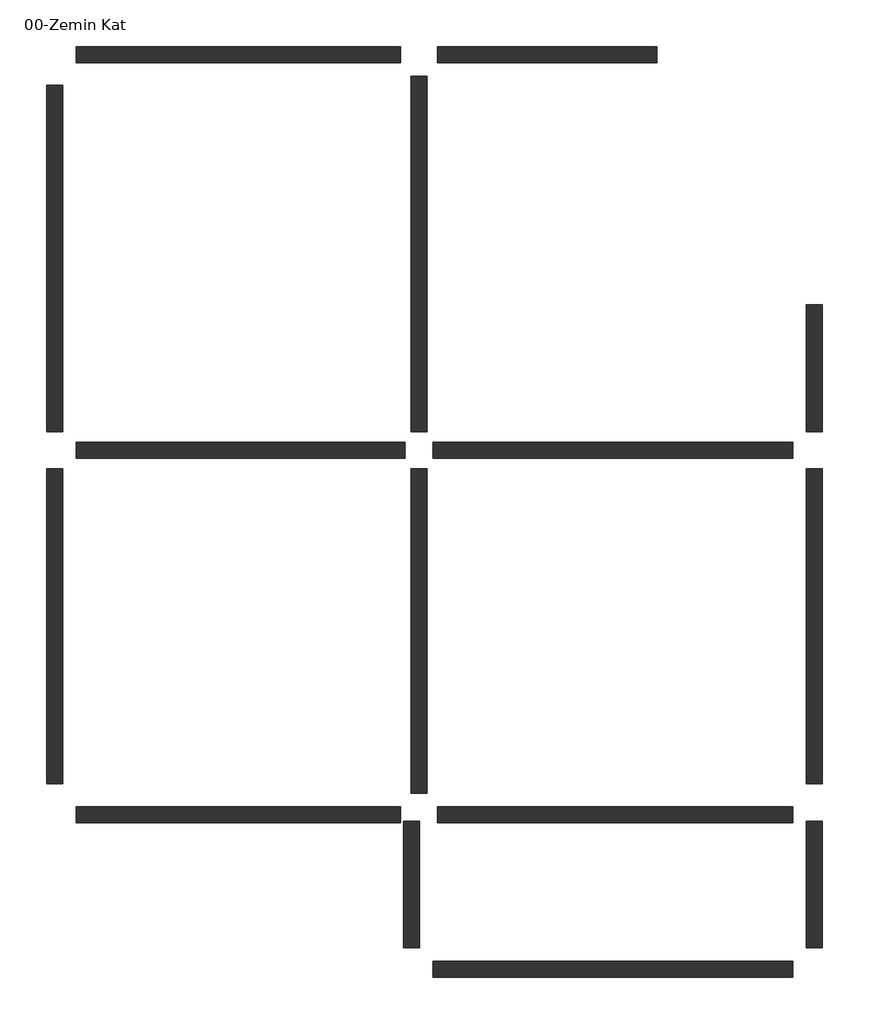
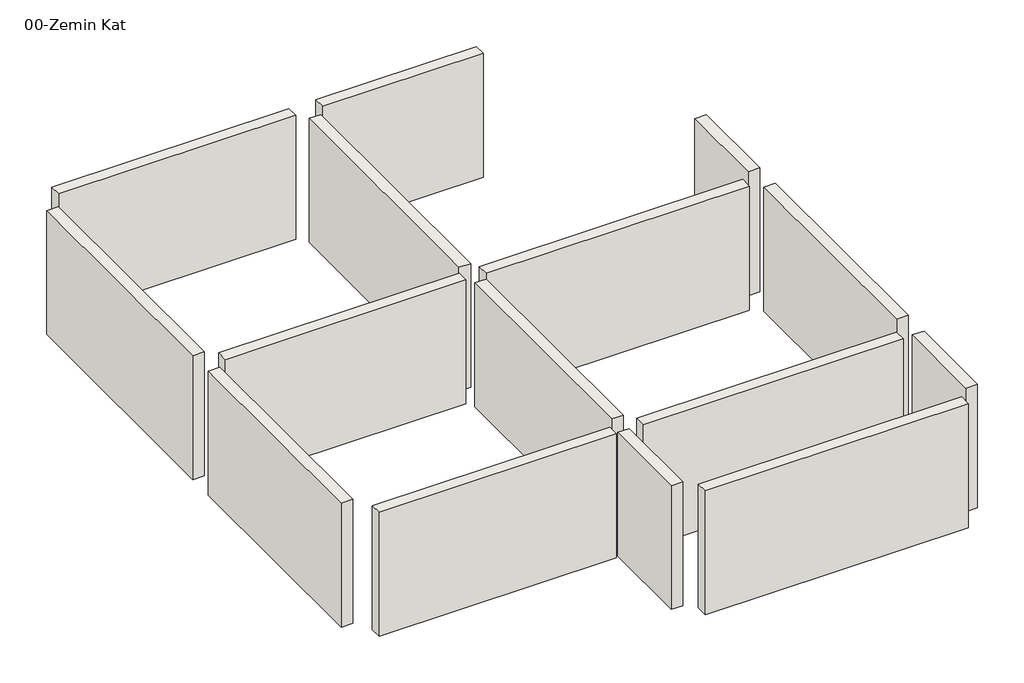
# One storey: 15 walls.
"""IFC4 building model written with IfcOpenShell, lengths in millimetres."""

import ifcopenshell
import ifcopenshell.guid

model = None  # the IFC model being written
_history = None  # IfcOwnerHistory: only IFC2X3 demands one
_inside = {}  # id of a spatial element -> (the spatial element, [elements in it])
_under = {}  # id of a project, library or spatial element -> (it, [spatial elements below it])
_declared = {}  # id of a project -> (the project, [libraries it declares])
_typed = {}  # id of a type object -> (the type object, [elements of that type])
_made_of = {}  # id of a material, layer set ... -> (it, [elements and type objects made of it])


def new_model(schema):
    """Start an empty IFC model of exactly this schema.

    Asked for "IFC4X3", IfcOpenShell would pick the latest addendum, in which some entities
    have other attributes; the version numbers below select the first issue.
    IFC2X3 requires an IfcOwnerHistory on every rooted entity: one is made here for all.
    """
    global model, _history
    if schema == "IFC4X3":
        model = ifcopenshell.file(schema_version=(4, 3, 0, 0))
    else:
        model = ifcopenshell.file(schema=schema)
    _inside.clear()
    _under.clear()
    _declared.clear()
    _typed.clear()
    _made_of.clear()
    _history = None
    if model.schema == "IFC2X3":
        org = make("IfcOrganization", Name="unknown")
        user = make(
            "IfcPersonAndOrganization",
            ThePerson=make("IfcPerson", FamilyName="unknown"),
            TheOrganization=org,
        )
        app = make(
            "IfcApplication",
            ApplicationDeveloper=org,
            Version="unknown",
            ApplicationFullName="unknown",
            ApplicationIdentifier="unknown",
        )
        _history = make(
            "IfcOwnerHistory",
            OwningUser=user,
            OwningApplication=app,
            ChangeAction="ADDED",
            CreationDate=0,
        )
    return model


def make(cls, **values):
    """One entity of the class cls with the attributes given. An attribute that is None is left unset."""
    return model.create_entity(
        cls, **{name: value for name, value in values.items() if value is not None}
    )


def rooted(cls, **values):
    """An entity with a GlobalId (a new one), such as an element, a storey or a relation."""
    return make(cls, GlobalId=ifcopenshell.guid.new(), OwnerHistory=_history, **values)


def si_unit(unit_type, name, prefix=None):
    """IfcSIUnit, for example si_unit("LENGTHUNIT", "METRE", prefix="MILLI")."""
    return make("IfcSIUnit", UnitType=unit_type, Prefix=prefix, Name=name)


def assignment(units):
    """IfcUnitAssignment: the units of a project."""
    return None if units is None else make("IfcUnitAssignment", Units=units)


def point(xyz):
    """IfcCartesianPoint."""
    return None if xyz is None else make("IfcCartesianPoint", Coordinates=xyz)


def direction(xyz):
    """IfcDirection."""
    return None if xyz is None else make("IfcDirection", DirectionRatios=xyz)


def frame(location, z_axis=None, x_axis=None):
    """IfcAxis2Placement3D, a coordinate frame: its origin and axes. An axis left out is left unset."""
    return make(
        "IfcAxis2Placement3D",
        Location=point(location),
        Axis=direction(z_axis),
        RefDirection=direction(x_axis),
    )


def origin():
    """The frame at (0, 0, 0) with its axes left unset."""
    return frame((0.0, 0.0, 0.0))


def place(relative_to, where):
    """IfcLocalPlacement: puts the frame where relative to a parent placement (None: the world)."""
    return make(
        "IfcLocalPlacement", PlacementRelTo=relative_to, RelativePlacement=where
    )


def context(
    kind, dimensions, precision=None, world=None, true_north=None, identifier=None
):
    """IfcGeometricRepresentationContext, for example the 3D "Model" context."""
    return make(
        "IfcGeometricRepresentationContext",
        ContextIdentifier=identifier,
        ContextType=kind,
        CoordinateSpaceDimension=dimensions,
        Precision=precision,
        WorldCoordinateSystem=world,
        TrueNorth=true_north,
    )


def project(units=None, contexts=None):
    """IfcProject with its units and contexts."""
    return rooted(
        "IfcProject",
        Name="project",
        RepresentationContexts=contexts,
        UnitsInContext=assignment(units),
    )


def spatial(cls, under=None, at=None, **own):
    """A site, building, storey or space (cls), placed at a placement, below another one or the project."""
    s = rooted(cls, ObjectPlacement=at, **own)
    if under is not None:
        _under.setdefault(under.id(), (under, []))[1].append(s)
    return s


def polyline(points):
    """IfcPolyline through the points."""
    return make("IfcPolyline", Points=[point(p) for p in points])


def outline(outer, holes=None, kind="AREA"):
    """IfcArbitraryClosedProfileDef: a profile drawn as a closed curve; with holes, ...WithVoids."""
    if holes is None:
        return make("IfcArbitraryClosedProfileDef", ProfileType=kind, OuterCurve=outer)
    return make(
        "IfcArbitraryProfileDefWithVoids",
        ProfileType=kind,
        OuterCurve=outer,
        InnerCurves=holes,
    )


def extrude(swept, where, along, depth):
    """IfcExtrudedAreaSolid: the profile swept, set in the frame where, extruded along a direction by depth."""
    return make(
        "IfcExtrudedAreaSolid",
        SweptArea=swept,
        Position=where,
        ExtrudedDirection=direction(along),
        Depth=depth,
    )


def shape(context_of_items, identifier, shape_type, items):
    """IfcShapeRepresentation: the items that make up one representation, for example the "Body"."""
    return make(
        "IfcShapeRepresentation",
        ContextOfItems=context_of_items,
        RepresentationIdentifier=identifier,
        RepresentationType=shape_type,
        Items=items,
    )


def made_of(thing, what):
    """Note that an element or type object is made of a material, layer set ...; save() writes the relation."""
    if what is not None:
        _made_of.setdefault(what.id(), (what, []))[1].append(thing)
    return thing


def element(
    cls,
    number,
    at=None,
    inside=None,
    cuts=None,
    type_object=None,
    material=None,
    context=None,
    identifier="Body",
    shape_type=None,
    held_by="IfcProductDefinitionShape",
    body=None,
    shapes=None,
    **own,
):
    """One element of the class cls, such as IfcWall. Its Tag is "e" and its number.

    at: its placement. inside: the storey or other place that contains it. cuts: it is an
    opening in that element (IfcRelVoidsElement). A single representation is given by context,
    identifier, shape_type and body (its items); several are given by shapes. held_by: the class
    of the entity that holds the representations. save() writes the other relations.
    """
    e = rooted(cls, Tag="e%d" % number, ObjectPlacement=at, **own)
    if body is not None:
        shapes = [shape(context, identifier, shape_type, body)]
    if shapes is not None:
        e.Representation = make(held_by, Representations=shapes)
    if inside is not None:
        _inside.setdefault(inside.id(), (inside, []))[1].append(e)
    if cuts is not None:
        rooted(
            "IfcRelVoidsElement", RelatingBuildingElement=cuts, RelatedOpeningElement=e
        )
    if type_object is not None:
        _typed.setdefault(type_object.id(), (type_object, []))[1].append(e)
    return made_of(e, material)


def aggregate(whole, parts):
    """IfcRelAggregates: a whole, such as a stair, and the parts it consists of."""
    return rooted("IfcRelAggregates", RelatingObject=whole, RelatedObjects=parts)


def save(model, path):
    """Write the relations noted so far, then the file.

    IfcRelAggregates (storeys below a building ...), IfcRelContainedInSpatialStructure (elements
    in a storey), IfcRelDefinesByType, IfcRelAssociatesMaterial and IfcRelDeclares: one each for
    every whole, place, type object, material and project.
    """
    for whole, parts in _under.values():
        aggregate(whole, parts)
    for where, things in _inside.values():
        rooted(
            "IfcRelContainedInSpatialStructure",
            RelatedElements=things,
            RelatingStructure=where,
        )
    for kind, things in _typed.values():
        rooted("IfcRelDefinesByType", RelatedObjects=things, RelatingType=kind)
    for what, things in _made_of.values():
        rooted("IfcRelAssociatesMaterial", RelatedObjects=things, RelatingMaterial=what)
    for by, libraries in _declared.values():
        rooted("IfcRelDeclares", RelatingContext=by, RelatedDefinitions=libraries)
    model.write(path)


model = new_model("IFC4")

# Units and contexts
model_context = context("Model", 3, world=origin())
ifc_project = project(units=[si_unit("LENGTHUNIT", "METRE", prefix="MILLI")], contexts=[model_context])

# Site, building, storey
site = spatial("IfcSite", under=ifc_project)
building = spatial("IfcBuilding", under=site)
storey = spatial("IfcBuildingStorey", under=building, Name="00-Zemin Kat", Elevation=93780.0)

# Walls
placement = place(None, origin())
element("IfcWall", 1, ObjectType="1.5BY-1.5SV-20BR-1.5-1.5BY", at=placement, inside=storey, context=model_context, shape_type="SweptSolid", body=[
    extrude(outline(polyline([(5700.0, 14770.0), (450.0, 14770.0), (450.0, 15030.0), (5700.0, 15030.0), (5700.0, 14770.0)])), frame((0.0, 0.0, 93780.0), z_axis=(0.0, 0.0, 1.0), x_axis=(1.0, 0.0, 0.0)), (0.0, 0.0, 1.0), 2900.0),
])
element("IfcWall", 2, ObjectType="1.5BY-1.5SV-20BR-1.5-1.5BY", at=placement, inside=storey, context=model_context, shape_type="SweptSolid", body=[
    extrude(outline(polyline([(9850.0, 14770.0), (6300.0, 14770.0), (6300.0, 15030.0), (9850.0, 15030.0), (9850.0, 14770.0)])), frame((0.0, 0.0, 93780.0), z_axis=(0.0, 0.0, 1.0), x_axis=(1.0, 0.0, 0.0)), (0.0, 0.0, 1.0), 2900.0),
])
element("IfcWall", 3, ObjectType="1.5BY-1.5SV-20BR-1.5-1.5BY", at=placement, inside=storey, context=model_context, shape_type="SweptSolid", body=[
    extrude(outline(polyline([(12270.0, 8800.0), (12270.0, 10850.0), (12530.0, 10850.0), (12530.0, 8800.0), (12270.0, 8800.0)])), frame((0.0, 0.0, 93780.0), z_axis=(0.0, 0.0, 1.0), x_axis=(1.0, 0.0, 0.0)), (0.0, 0.0, 1.0), 2900.0),
])
element("IfcWall", 4, ObjectType="1.5BY-1.5SV-20BR-1.5-1.5BY", at=placement, inside=storey, context=model_context, shape_type="SweptSolid", body=[
    extrude(outline(polyline([(12270.0, 3100.0), (12270.0, 8200.0), (12530.0, 8200.0), (12530.0, 3100.0), (12270.0, 3100.0)])), frame((0.0, 0.0, 93780.0), z_axis=(0.0, 0.0, 1.0), x_axis=(1.0, 0.0, 0.0)), (0.0, 0.0, 1.0), 2900.0),
])
element("IfcWall", 5, ObjectType="1.5BY-1.5SV-20BR-1.5-1.5BY", at=placement, inside=storey, context=model_context, shape_type="SweptSolid", body=[
    extrude(outline(polyline([(12270.0, 450.0), (12270.0, 2500.0), (12530.0, 2500.0), (12530.0, 450.0), (12270.0, 450.0)])), frame((0.0, 0.0, 93780.0), z_axis=(0.0, 0.0, 1.0), x_axis=(1.0, 0.0, 0.0)), (0.0, 0.0, 1.0), 2900.0),
])
element("IfcWall", 6, ObjectType="1.5BY-1.5SV-20BR-1.5-1.5BY", at=placement, inside=storey, context=model_context, shape_type="SweptSolid", body=[
    extrude(outline(polyline([(6225.0, 230.0), (12050.0, 230.0), (12050.0, -30.0), (6225.0, -30.0), (6225.0, 230.0)])), frame((0.0, 0.0, 93780.0), z_axis=(0.0, 0.0, 1.0), x_axis=(1.0, 0.0, 0.0)), (0.0, 0.0, 1.0), 2900.0),
])
element("IfcWall", 7, ObjectType="1.5BY-1.5SV-20BR-1.5-1.5BY", at=placement, inside=storey, context=model_context, shape_type="SweptSolid", body=[
    extrude(outline(polyline([(6005.0, 2500.0), (6005.0, 450.0), (5745.0, 450.0), (5745.0, 2500.0), (6005.0, 2500.0)])), frame((0.0, 0.0, 93780.0), z_axis=(0.0, 0.0, 1.0), x_axis=(1.0, 0.0, 0.0)), (0.0, 0.0, 1.0), 2900.0),
])
element("IfcWall", 8, ObjectType="1.5BY-1.5SV-20BR-1.5-1.5BY", at=placement, inside=storey, context=model_context, shape_type="SweptSolid", body=[
    extrude(outline(polyline([(450.0, 2730.0), (5700.0, 2730.0), (5700.0, 2470.0), (450.0, 2470.0), (450.0, 2730.0)])), frame((0.0, 0.0, 93780.0), z_axis=(0.0, 0.0, 1.0), x_axis=(1.0, 0.0, 0.0)), (0.0, 0.0, 1.0), 2900.0),
])
element("IfcWall", 9, ObjectType="1.5BY-1.5SV-20BR-1.5-1.5BY", at=placement, inside=storey, context=model_context, shape_type="SweptSolid", body=[
    extrude(outline(polyline([(230.0, 8200.0), (230.0, 3100.0), (-30.0, 3100.0), (-30.0, 8200.0), (230.0, 8200.0)])), frame((0.0, 0.0, 93780.0), z_axis=(0.0, 0.0, 1.0), x_axis=(1.0, 0.0, 0.0)), (0.0, 0.0, 1.0), 2900.0),
])
element("IfcWall", 10, ObjectType="1.5BY-1.5SV-20BR-1.5-1.5BY", at=placement, inside=storey, context=model_context, shape_type="SweptSolid", body=[
    extrude(outline(polyline([(230.0, 14400.0), (230.0, 8800.0), (-30.0, 8800.0), (-30.0, 14400.0), (230.0, 14400.0)])), frame((0.0, 0.0, 93780.0), z_axis=(0.0, 0.0, 1.0), x_axis=(1.0, 0.0, 0.0)), (0.0, 0.0, 1.0), 2900.0),
])
element("IfcWall", 11, ObjectType="1.5BY-1.5SV-20BR-1.5-1.5BY", at=placement, inside=storey, context=model_context, shape_type="SweptSolid", body=[
    extrude(outline(polyline([(6300.0, 2730.0), (12050.0, 2730.0), (12050.0, 2470.0), (6300.0, 2470.0), (6300.0, 2730.0)])), frame((0.0, 0.0, 93780.0), z_axis=(0.0, 0.0, 1.0), x_axis=(1.0, 0.0, 0.0)), (0.0, 0.0, 1.0), 2900.0),
])
element("IfcWall", 12, ObjectType="1.5BY-1.5SV-20BR-1.5-1.5BY", at=placement, inside=storey, context=model_context, shape_type="SweptSolid", body=[
    extrude(outline(polyline([(6130.0, 8200.0), (6130.0, 2950.0), (5870.0, 2950.0), (5870.0, 8200.0), (6130.0, 8200.0)])), frame((0.0, 0.0, 93780.0), z_axis=(0.0, 0.0, 1.0), x_axis=(1.0, 0.0, 0.0)), (0.0, 0.0, 1.0), 2900.0),
])
element("IfcWall", 13, ObjectType="1.5BY-1.5SV-20BR-1.5-1.5BY", at=placement, inside=storey, context=model_context, shape_type="SweptSolid", body=[
    extrude(outline(polyline([(6130.0, 14550.0), (6130.0, 8800.0), (5870.0, 8800.0), (5870.0, 14550.0), (6130.0, 14550.0)])), frame((0.0, 0.0, 93780.0), z_axis=(0.0, 0.0, 1.0), x_axis=(1.0, 0.0, 0.0)), (0.0, 0.0, 1.0), 2900.0),
])
element("IfcWall", 14, ObjectType="1.5BY-1.5SV-20BR-1.5-1.5BY", at=placement, inside=storey, context=model_context, shape_type="SweptSolid", body=[
    extrude(outline(polyline([(5775.0, 8370.0), (450.0, 8370.0), (450.0, 8630.0), (5775.0, 8630.0), (5775.0, 8370.0)])), frame((0.0, 0.0, 93780.0), z_axis=(0.0, 0.0, 1.0), x_axis=(1.0, 0.0, 0.0)), (0.0, 0.0, 1.0), 2900.0),
])
element("IfcWall", 15, ObjectType="1.5BY-1.5SV-20BR-1.5-1.5BY", at=placement, inside=storey, context=model_context, shape_type="SweptSolid", body=[
    extrude(outline(polyline([(12050.0, 8370.0), (6225.0, 8370.0), (6225.0, 8630.0), (12050.0, 8630.0), (12050.0, 8370.0)])), frame((0.0, 0.0, 93780.0), z_axis=(0.0, 0.0, 1.0), x_axis=(1.0, 0.0, 0.0)), (0.0, 0.0, 1.0), 2900.0),
])

save(model, "model.ifc")

# Revit data of these elements
# Project information
#   Project Issue Date = "Issue Date"
#   Project Status = "Project Status"
#   Client Name = "Owner"
#   Project Address = "Enter address here"
#   Project Name = "Project Name"
#   Project Number = "0001"
# Type "1.5BY-1.5SV-20BR-1.5-1.5BY"
#   Layers, outside or top first: 15 mm "Parking Stripe" (function 5); 15 mm "Siva" (function 4); 200 mm "tugla" (function 1); 15 mm "Siva" (function 4); 15 mm "Parking Stripe" (function 5)
# Elements 1, 2, 3, 4, 5, 6, 7, 8, 9, 10, 11, 12, 13, 14, 15 (IfcWall, "1.5BY-1.5SV-20BR-1.5-1.5BY")
#   Top Offset = -600 mm
#   Base Offset = 0 mm
#   wall height = 2900 mm
#   Phase Created = New Construction
#   Base Constraint = 00-Zemin Kat
#   Top Constraint = 01-Birinci Kat
#   Materials on its faces: "Default Wall", "Parking Stripe"
# Materials
#   "Parking Stripe": class "Paint", colour RGB 250 250 91, transparency 0, Cost = 0
#   "Siva": class "Generic", colour RGB 249 249 249, transparency 0, Description = "Gypsum Wall Board", Cost = 0
#   "tugla": class "Masonry", colour RGB 170 100 105, transparency 0, Description = "Common brick", Cost = 0
#   "Default Wall": class "Miscellaneous", colour RGB 128 128 128, transparency 0, Cost = 0
